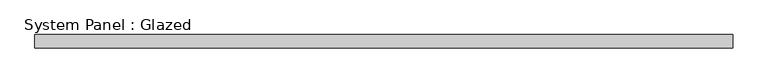
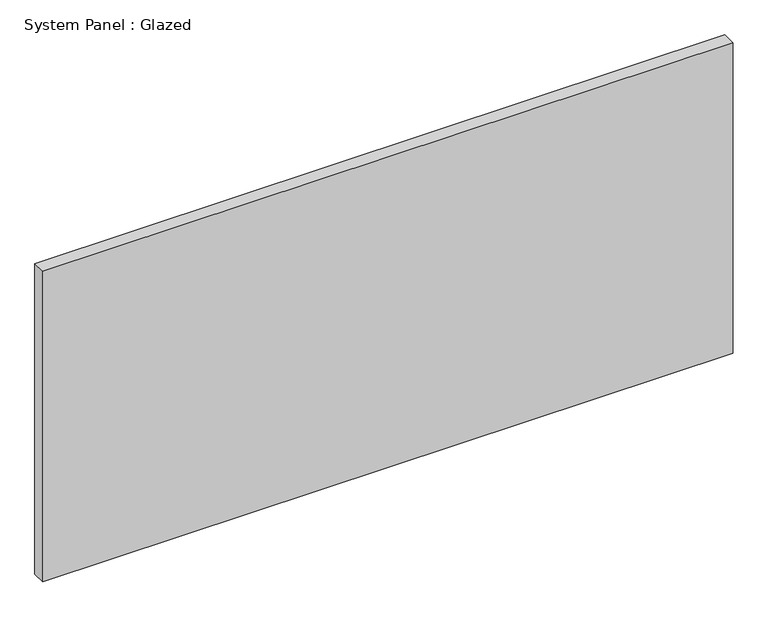
"""IFC4 building model written with IfcOpenShell, lengths in millimetres: plate geometry, System Panel : Glazed."""

from ifc_helpers import new_model, si_unit, origin, origin_with_axes, place, context, project, spatial, polyline, outline, extrude, source, transform, mapped, element, save


def system_panel_glazed_f3674cde(model_context):
    return source(origin(), model_context, "Body", "SweptSolid", [
        extrude(outline(polyline([(654.05, 19.05), (-654.05, 19.05), (-654.05, 44.45), (654.05, 44.45), (654.05, 19.05)])), origin_with_axes(), (0.0, 0.0, 1.0), 622.3),
    ])


if __name__ == "__main__":
    model = new_model("IFC4")
    model_context = context("Model", 3, world=origin())
    ifc_project = project(units=[si_unit("LENGTHUNIT", "METRE", prefix="MILLI")], contexts=[model_context])
    site = spatial("IfcSite", under=ifc_project)
    building = spatial("IfcBuilding", under=site)
    placement = place(None, origin())
    system_panel_glazed_shape = system_panel_glazed_f3674cde(model_context)
    element("IfcPlate", 1, ObjectType="System Panel : Glazed", at=placement, inside=building, context=model_context, shape_type="MappedRepresentation", body=[
        mapped(system_panel_glazed_shape, transform((0.0, 0.0, 0.0), x_axis=(1.0, 0.0, 0.0), y_axis=(0.0, 1.0, 0.0), z_axis=(0.0, 0.0, 1.0))),
    ])
    save(model, "model.ifc")

# Revit data of these elements
# Element 1 (IfcPlate, "System Panel : Glazed")
#   Materials on its faces: "Glass"
# Materials
#   "Glass": class "Glass", colour RGB 0 128 192, transparency 0.75
